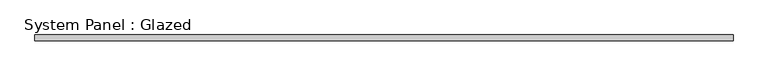
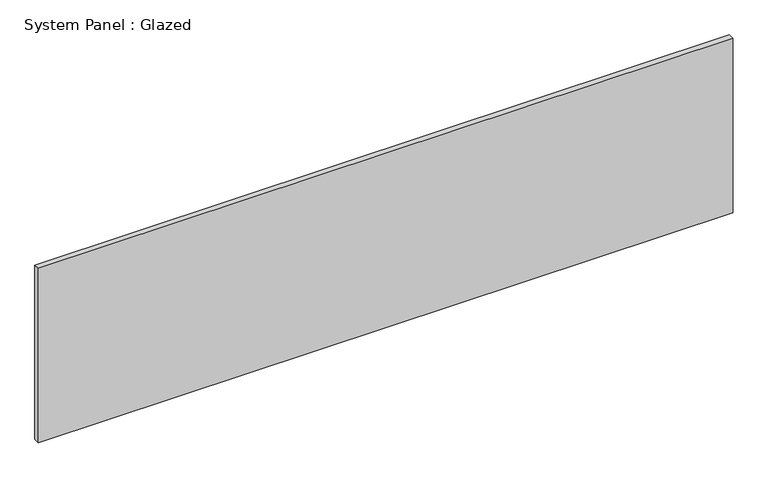
"""IFC4 building model written with IfcOpenShell, lengths in millimetres: plate geometry, System Panel : Glazed."""

from ifc_helpers import new_model, si_unit, origin, origin_with_axes, place, context, project, spatial, polyline, outline, extrude, source, transform, mapped, element, save


def system_panel_glazed_b70978ba(model_context):
    return source(origin(), model_context, "Body", "SweptSolid", [
        extrude(outline(polyline([(1543.05, -44.45), (-1543.05, -44.45), (-1543.05, -19.05), (1543.05, -19.05), (1543.05, -44.45)])), origin_with_axes(), (0.0, 0.0, 1.0), 819.15),
    ])


if __name__ == "__main__":
    model = new_model("IFC4")
    model_context = context("Model", 3, world=origin())
    ifc_project = project(units=[si_unit("LENGTHUNIT", "METRE", prefix="MILLI")], contexts=[model_context])
    site = spatial("IfcSite", under=ifc_project)
    building = spatial("IfcBuilding", under=site)
    placement = place(None, origin())
    system_panel_glazed_shape = system_panel_glazed_b70978ba(model_context)
    element("IfcPlate", 1, ObjectType="System Panel : Glazed", at=placement, inside=building, context=model_context, shape_type="MappedRepresentation", body=[
        mapped(system_panel_glazed_shape, transform((0.0, 0.0, 0.0), x_axis=(1.0, 0.0, 0.0), y_axis=(0.0, 1.0, 0.0), z_axis=(0.0, 0.0, 1.0))),
    ])
    save(model, "model.ifc")

# Revit data of these elements
# Type "System Panel : Glazed"
#   Construction Type Id = "GSP4R"
#   Analytic Construction = "1/8 in Pilkington single glazing"
#   Visual Light Transmittance = 0.9
#   Solar Heat Gain Coefficient = 0.86
#   Heat Transfer Coefficient (U) = 1.18115 BTU/(h·ft²·°F)
#   Define Thermal Properties by = 1
# Element 1 (IfcPlate, "System Panel : Glazed")
#   Materials on its faces: "Glass"
# Materials
#   "Glass": class "Glass", colour RGB 0 128 192, transparency 0.75, Description = "Soda Lime Glass", Cost = 0
